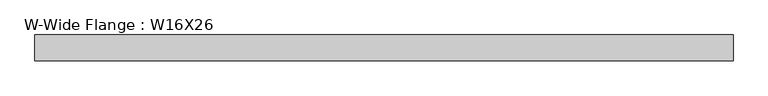
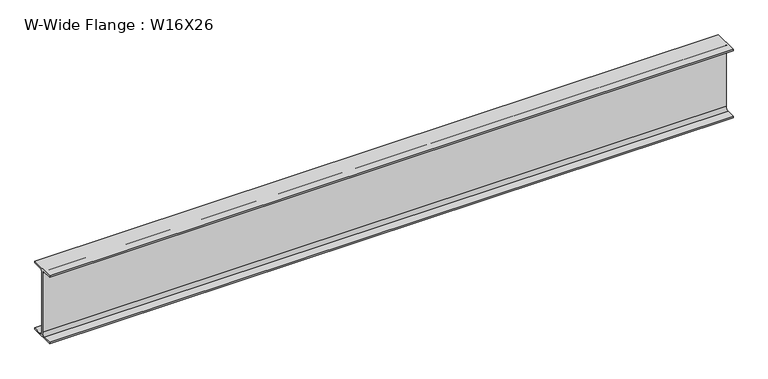
"""IFC4 building model written with IfcOpenShell, lengths in millimetres: beam geometry, W-Wide Flange : W16X26."""

from ifc_helpers import new_model, si_unit, point, frame, frame_2d, origin, place, context, project, spatial, polyline, circle_curve, trimmed, segment, composite_curve, outline, extrude, source, transform, mapped, element, save


def w_wide_flange_w16x26_af4b12ba(model_context):
    return source(origin(), model_context, "Body", "SweptSolid", [
        extrude(outline(composite_curve([segment(polyline([(-69.85, -190.5496094), (-21.43125, -190.5496094)]), True, "CONTINUOUS"), segment(trimmed(circle_curve(frame_2d((-21.43125, -172.2933594)), 18.25625), [point((-21.43125, -190.5496094))], [point((-3.175, -172.2933594))], True, "CARTESIAN"), True, "CONTINUOUS"), segment(polyline([(-3.175, -172.2933594), (-3.175, 172.2933594)]), True, "CONTINUOUS"), segment(trimmed(circle_curve(frame_2d((-21.43125, 172.2933594)), 18.25625), [point((-3.175, 172.2933594))], [point((-21.43125, 190.5496094))], True, "CARTESIAN"), True, "CONTINUOUS"), segment(polyline([(-21.43125, 190.5496094), (-69.85, 190.5496094), (-69.85, 199.2808594), (69.85, 199.2808594), (69.85, 190.5496094), (21.43125, 190.5496094)]), True, "CONTINUOUS"), segment(trimmed(circle_curve(frame_2d((21.43125, 172.2933594)), 18.25625), [point((21.43125, 190.5496094))], [point((3.175, 172.2933594))], True, "CARTESIAN"), True, "CONTINUOUS"), segment(polyline([(3.175, 172.2933594), (3.175, -172.2933594)]), True, "CONTINUOUS"), segment(trimmed(circle_curve(frame_2d((21.43125, -172.2933594)), 18.25625), [point((3.175, -172.2933594))], [point((21.43125, -190.5496094))], True, "CARTESIAN"), True, "CONTINUOUS"), segment(polyline([(21.43125, -190.5496094), (69.85, -190.5496094), (69.85, -199.2808594), (-69.85, -199.2808594), (-69.85, -190.5496094)]), True, "CONTINUOUS")], self_intersect=False)), frame((-1892.3, 0.0, 0.0), z_axis=(1.0, 0.0, 0.0), x_axis=(0.0, 1.0, 0.0)), (0.0, 0.0, 1.0), 3778.3988281),
    ])


if __name__ == "__main__":
    model = new_model("IFC4")
    model_context = context("Model", 3, world=origin())
    ifc_project = project(units=[si_unit("LENGTHUNIT", "METRE", prefix="MILLI")], contexts=[model_context])
    site = spatial("IfcSite", under=ifc_project)
    building = spatial("IfcBuilding", under=site)
    placement = place(None, origin())
    w_wide_flange_w16x26_shape = w_wide_flange_w16x26_af4b12ba(model_context)
    element("IfcBeam", 1, ObjectType="W-Wide Flange : W16X26", at=placement, inside=building, context=model_context, shape_type="MappedRepresentation", body=[
        mapped(w_wide_flange_w16x26_shape, transform((0.0, 0.0, 0.0), x_axis=(1.0, 0.0, 0.0), y_axis=(0.0, 1.0, 0.0), z_axis=(0.0, 0.0, 1.0))),
    ])
    save(model, "model.ifc")

# Revit data of these elements
# Type "W-Wide Flange : W16X26"
#   Assembly Code = "B10"
#   W = 26
#   Start Extension Calculation [instance default] = 10' - 0"
#   Start Extension [instance default] = -0' - 0 1/2"
#   End Extension Calculation [instance default] = 10' - 0"
#   End Extension [instance default] = -0' - 0 1/2"
#   Length [instance default] = 5' - 0"
#   bf = 0' - 5 1/2"
#   d = 1' - 3 177/256"
#   k = 0' - 1 1/16"
#   k2 = 0' - 0 23/32"
#   tf = 0' - 0 11/32"
#   tw = 0' - 0 1/4"
#   A = 0.05 SF
#   Beam Material [instance default] = Metal - Steel - ASTM A992
# Element 1 (IfcBeam, "W-Wide Flange : W16X26")
#   Materials on its faces: "Metal - Steel - ASTM A992"
# Materials
#   "Metal - Steel - ASTM A992": class "Metal", colour RGB 128 0 0, transparency 0
